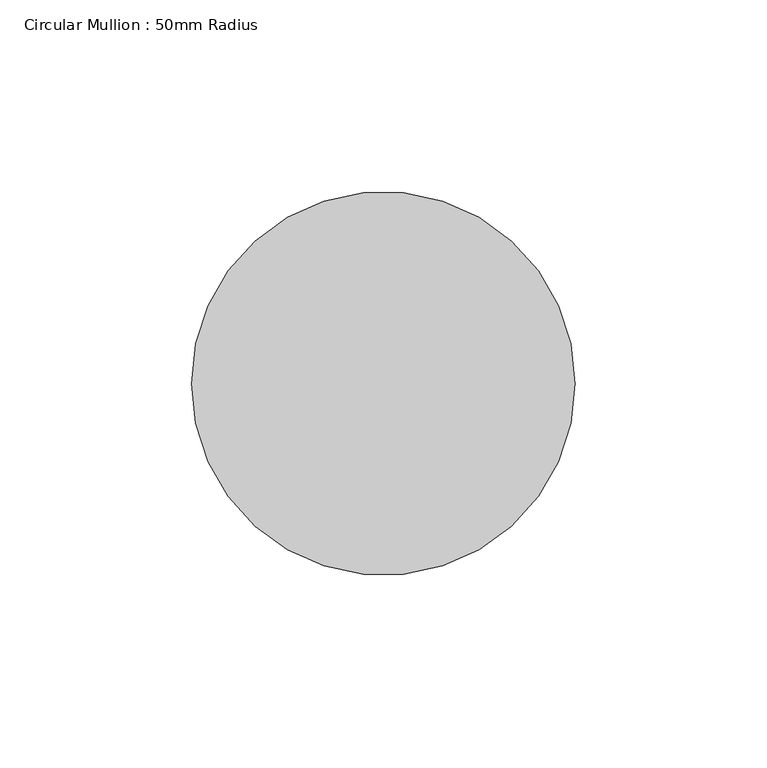
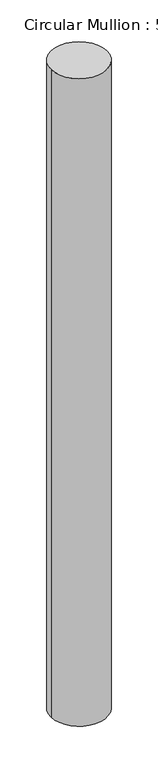
"""IFC4 building model written with IfcOpenShell, lengths in millimetres: member geometry, Circular Mullion : 50mm Radius."""

from ifc_helpers import new_model, si_unit, point, frame, origin, origin_2d, place, context, project, spatial, circle_curve, trimmed, segment, composite_curve, outline, extrude, source, transform, mapped, element, save


def circular_mullion_50mm_radius_eb8b356c(model_context):
    return source(origin(), model_context, "Body", "SweptSolid", [
        extrude(outline(composite_curve([segment(trimmed(circle_curve(origin_2d(), 50.0), [point((50.0, 0.0))], [point((-50.0, 0.0))], False, "CARTESIAN"), True, "CONTINUOUS"), segment(trimmed(circle_curve(origin_2d(), 50.0), [point((-50.0, 0.0))], [point((50.0, 0.0))], False, "CARTESIAN"), True, "CONTINUOUS")], self_intersect=False)), frame((0.0, 0.0, -1225.1266399), z_axis=(0.0, 0.0, 1.0), x_axis=(1.0, 0.0, 0.0)), (0.0, 0.0, 1.0), 1225.1266399),
    ])


if __name__ == "__main__":
    model = new_model("IFC4")
    model_context = context("Model", 3, world=origin())
    ifc_project = project(units=[si_unit("LENGTHUNIT", "METRE", prefix="MILLI")], contexts=[model_context])
    site = spatial("IfcSite", under=ifc_project)
    building = spatial("IfcBuilding", under=site)
    placement = place(None, origin())
    circular_mullion_50mm_radius_shape = circular_mullion_50mm_radius_eb8b356c(model_context)
    element("IfcMember", 1, ObjectType="Circular Mullion : 50mm Radius", at=placement, inside=building, context=model_context, shape_type="MappedRepresentation", body=[
        mapped(circular_mullion_50mm_radius_shape, transform((0.0, 0.0, 0.0), x_axis=(1.0, 0.0, 0.0), y_axis=(0.0, 1.0, 0.0), z_axis=(0.0, 0.0, 1.0))),
    ])
    save(model, "model.ifc")

# Revit data of these elements
# Type "Circular Mullion : 50mm Radius"
#   built-in parameter 1007350 = 0.164042 (stored number, unit not read)
# Element 1 (IfcMember, "Circular Mullion : 50mm Radius")
#   Materials on its faces: "Aluminium"
# Materials
#   "Aluminium": class "Metal", colour RGB 247 247 247, transparency 0, Description = "Aluminium 6061", Cost = 0
